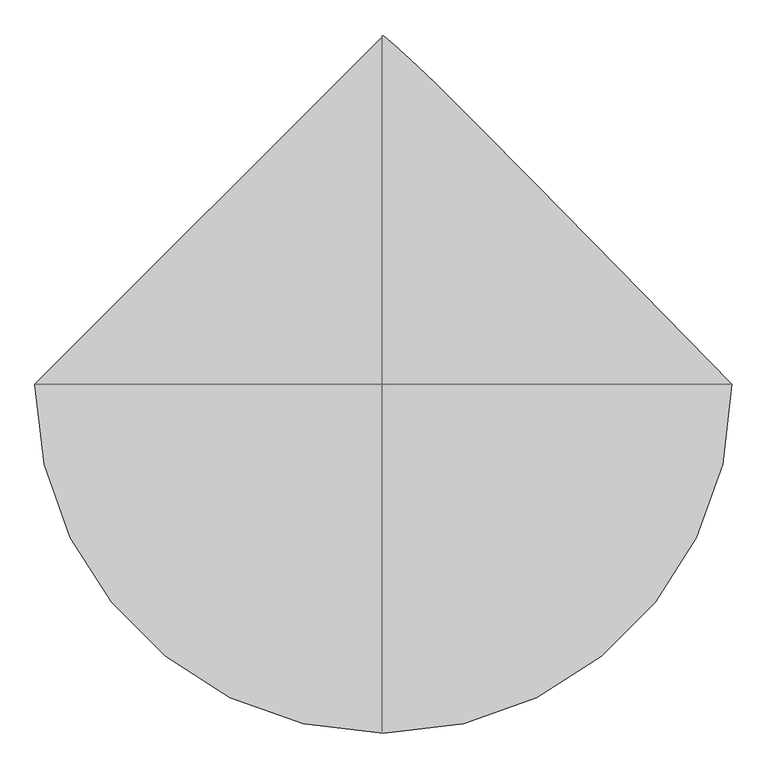
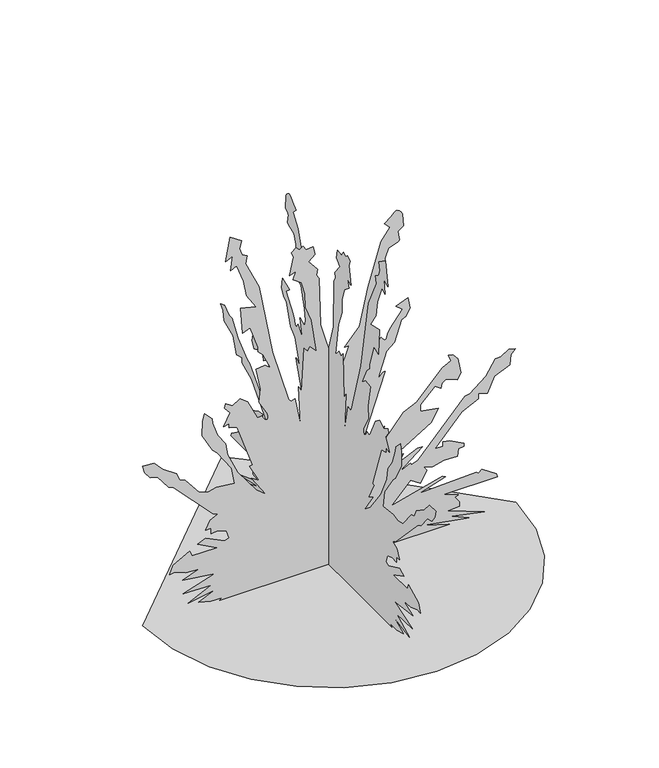
"""IFC4 building model written with IfcOpenShell, lengths in millimetres: proxy geometry, maiden grass 26738 : maiden grass 26738."""

from ifc_helpers import new_model, si_unit, origin, place, context, project, spatial, triangles, source, transform, mapped, element, save


def entourage_51d93d44(model_context):
    return source(origin(), model_context, "Body", "Tessellation", [
        triangles([(-822.1126825, 0.0, 0.0001374), (-800.3786167, -188.373858, 0.0001374), (-738.480578, -361.3651156, 0.0001374), (-641.3745867, -514.0173532, 0.0001374), (-514.0174622, -641.374732, 0.0001374), (-361.365043, -738.4805054, 0.0001374), (-188.3737671, -800.378544, 0.0001374), (3.59e-05, -822.1126825, 0.0001374), (188.3739125, -800.3786167, 0.0001374), (361.3651883, -738.480578, 0.0001374), (514.0174622, -641.3745867, 0.0001374), (641.3748047, -514.0174622, 0.0001374), (738.4805054, -361.365043, 0.0001374), (800.378544, -188.373749, 0.0001374), (822.1126825, 7.19e-05, 0.0001374), (554.9441065, 274.0493697, 0.0001374), (356.8788342, 475.8195757, 0.0001374), (216.3996546, 617.3571573, 0.0001374), (121.9894107, 710.7087994, 0.0001374), (62.1308551, 767.9210049, 0.0001374), (25.3067606, 801.0401316, 0.0001374), (-0.0001078, 822.1126825, 0.0001374), (-486.0236403, 7.81e-05, 0.9155915), (-471.7920599, 7.76e-05, 9.8343198), (-523.9165309, 7.76e-05, 9.7573804), (-575.3383922, 7.67e-05, 24.6529329), (-504.1805263, 7.48e-05, 56.6647099), (-622.6670803, 7.61e-05, 35.566252), (-521.099806, 7.32e-05, 83.8197293), (-644.3685173, 7.29e-05, 88.7502968), (-506.307395, 7.03e-05, 133.1254316), (-645.8895727, 6.92e-05, 151.363835), (-575.3383922, 6.76e-05, 177.5005391), (-633.4720894, 6.73e-05, 182.811861), (-682.2468012, 6.62e-05, 200.8128698), (-703.5376528, 6.64e-05, 197.2227365), (-688.7453144, 6.41e-05, 236.667331), (-614.7840586, 6.17e-05, 276.1118528), (-604.9224512, 6.32e-05, 251.4590335), (-494.8790591, 6.34e-05, 248.9685605), (-580.2687962, 6.06e-05, 295.8341047), (-545.7534247, 5.97e-05, 310.6258072), (-461.9305979, 6.2e-05, 271.1812672), (-442.4802589, 6.16e-05, 277.8612192), (-452.1878423, 5.96e-05, 312.2414789), (-492.5862848, 5.87e-05, 327.4185685), (-520.7920123, 5.89e-05, 323.5701842), (-521.099806, 5.73e-05, 350.0703109), (-545.7534247, 5.73e-05, 350.0703109), (-526.0308277, 5.5e-05, 389.5148872), (-491.515202, 5.41e-05, 404.3065716), (-513.2632931, 5.35e-05, 414.7085166), (-685.7770363, 4.26e-05, 596.5231456), (-707.8857159, 4.2e-05, 606.6573017), (-757.7759846, 3.82e-05, 670.5571804), (-790.6316099, 3.78e-05, 677.9690826), (-814.6804327, 3.58e-05, 711.7275599), (-821.8761417, 3.38e-05, 744.5156021), (-771.5802292, 3.4e-05, 740.8769434), (-734.9066683, 3.66e-05, 698.0076851), (-673.9536301, 3.91e-05, 655.7654961), (-659.1609283, 4.12e-05, 621.2515417), (-636.2393623, 4.16e-05, 613.9256081), (-573.062332, 4.63e-05, 535.429927), (-531.2541281, 4.7e-05, 522.9600486), (-496.445933, 4.65e-05, 532.501254), (-417.5538008, 4.7e-05, 522.6401553), (-431.8794525, 4.26e-05, 597.7539207), (-494.1621334, 3.7e-05, 691.4321417), (-515.1618327, 3.58e-05, 710.6897598), (-560.6032451, 3.08e-05, 794.7286709), (-559.6332461, 2.68e-05, 861.8978268), (-550.6847371, 2.5e-05, 892.4327362), (-516.1688933, 2.71e-05, 857.9187092), (-514.4276842, 2.84e-05, 836.1371899), (-492.5786181, 3.21e-05, 773.1969183), (-456.9999032, 3.53e-05, 719.8628918), (-448.1073864, 3.85e-05, 666.0661755), (-403.8973306, 4.42e-05, 569.7717261), (-322.5198123, 5.08e-05, 459.5990905), (-279.4932235, 5.29e-05, 424.0288053), (-341.7963246, 4.73e-05, 518.5882951), (-309.0772825, 4.85e-05, 497.987336), (-351.6489936, 4.37e-05, 579.3482491), (-338.6617049, 4.35e-05, 581.8069654), (-407.6923751, 3.18e-05, 779.0296291), (-442.2077102, 3.12e-05, 788.8907278), (-442.2077102, 3e-05, 808.6129978), (-466.8613289, 3.03e-05, 803.6824848), (-437.2769065, 2.71e-05, 857.9187092), (-461.9305979, 2.53e-05, 887.5020779), (-456.9999032, 2.41e-05, 907.2244205), (-427.4157715, 2.53e-05, 887.5020779), (-392.9001457, 2.41e-05, 907.2244205), (-361.3909862, 2.55e-05, 883.444622), (-319.5289701, 3.13e-05, 794.863619), (-316.5251201, 3.15e-05, 792.847681), (-312.9193082, 3.15e-05, 792.290593), (-308.9018935, 3.15e-05, 792.6843916), (-304.6633259, 3.13e-05, 793.5212591), (-300.3935829, 3.11e-05, 794.293523), (-296.2831507, 3.08e-05, 794.4932928), (-293.8821344, 3.1e-05, 789.7024515), (-291.6524922, 3.11e-05, 784.6016001), (-289.2939152, 3.13e-05, 779.6455799), (-286.5060222, 3.14e-05, 775.2894505), (-282.9887042, 3.16e-05, 771.9882711), (-278.4414163, 3.19e-05, 770.1969561), (-272.5639226, 3.23e-05, 770.3705647), (-270.4821274, 3.19e-05, 776.4802935), (-269.746798, 3.16e-05, 782.5422054), (-271.4178988, 3.09e-05, 794.5538269), (-309.0772825, 2.68e-05, 862.8492222), (-304.1468967, 2.32e-05, 922.0159595), (-323.8695119, 1.74e-05, 1020.6273823), (-284.423464, 1.71e-05, 1025.5578953), (-259.7697544, 1.82e-05, 1005.8357706), (-292.5143764, 1.4e-05, 1076.7667608), (-314.0080499, 1.27e-05, 1099.5164623), (-315.0547156, 1.15e-05, 1119.0795851), (-348.5233486, 5.3e-06, 1222.7807407), (-383.038502, 6.2e-06, 1207.9888384), (-391.1781941, -1e-06, 1327.8346481), (-323.8695119, 0.0, 1311.5309921), (-365.2547038, -3.9e-06, 1377.9884182), (-377.5616561, -8.2e-06, 1449.0455635), (-409.7759325, -1.31e-05, 1532.0531422), (-435.1933854, -1.24e-05, 1519.3450516), (-427.4157715, -1.61e-05, 1582.7118233), (-456.9999032, -1.53e-05, 1567.9204296), (-438.6445556, -2.17e-05, 1676.3998547), (-387.9694147, -1.97e-05, 1641.8788513), (-396.0815286, -1.75e-05, 1605.9381672), (-384.2218237, -1.56e-05, 1574.3406773), (-363.3155416, -1.5e-05, 1562.9896259), (-368.246309, -1.29e-05, 1528.4758896), (-309.0772825, -5.3e-06, 1400.2812435), (-250.6196225, 1.42e-05, 1073.5192846), (-180.2010283, 2.87e-05, 830.6251717), (-169.6161911, 2.95e-05, 817.4087545), (-151.2930636, 2.91e-05, 823.4046822), (-126.6192335, 3.68e-05, 694.4196774), (-136.5008433, 2.62e-05, 872.7103935), (-121.7086412, 2.76e-05, 848.0576105), (-111.8470156, 1.59e-05, 1045.2803106), (-97.0548044, 1.71e-05, 1025.5578953), (-84.6295182, 1.62e-05, 1040.6290684), (-57.6092516, 1.79e-05, 1010.7662109), (-79.5582798, 8.8e-06, 1163.7574539), (-104.4511553, 4.7e-06, 1232.6419121), (-107.5404289, 9e-07, 1296.0368797), (-123.4986664, -2.4e-06, 1352.177639), (-161.1545347, -4.1e-06, 1380.5586102), (-146.3623326, -6.2e-06, 1415.0727825), (-175.9469094, -5.6e-06, 1405.2116112), (-158.7234512, -1.03e-05, 1484.8167812), (-166.0854474, -1.17e-05, 1508.7534016), (-146.3623326, -1.26e-05, 1523.5452312), (-131.5704484, -1.17e-05, 1508.7534016), (-116.6065998, -1.25e-05, 1521.4754448), (-101.9855355, -1.11e-05, 1498.8923756), (-72.4009586, -1.14e-05, 1503.8230339), (-62.5394784, -9.1e-06, 1464.3783485), (-92.1240644, -7.6e-06, 1439.7256382), (-52.6780073, -4.7e-06, 1390.4200722), (-57.6092516, -3.2e-06, 1365.7670712), (-44.9584885, -2.1e-06, 1346.546006), (-40.1288097, 1.1e-05, 1128.143712), (16.3521246, 2.24e-05, 936.8077166), (25.6302442, 2.16e-05, 950.3199005), (46.3616142, 2.59e-05, 877.5758669), (85.383115, 1.94e-05, 986.1135006), (65.6596505, 1.94e-05, 986.1135006), (132.852038, 1.49e-05, 1062.0039265), (169.7376772, 4.9e-06, 1229.8971668), (228.245861, -6.6e-06, 1421.9566647), (267.8211162, -9.7e-06, 1474.2395199), (243.1672431, -1.11e-05, 1498.8923756), (272.0833378, -1.25e-05, 1521.3225471), (286.4673436, -1.31e-05, 1537.556876), (293.7374485, -1.35e-05, 1542.3155972), (297.4055931, -1.38e-05, 1543.2675739), (308.1376596, -1.27e-05, 1537.579549), (315.8437663, -1.16e-05, 1529.0826839), (321.0283699, -1.07e-05, 1518.2452641), (326.6370392, -7.7e-06, 1460.8509476), (306.7311321, -7.7e-06, 1447.4507481), (304.3311514, -7.7e-06, 1444.519241), (302.7936726, -7.7e-06, 1441.4505329), (309.1859605, -6.2e-06, 1402.4600349), (307.1584316, -5.9e-06, 1398.4450184), (302.9130694, -5.6e-06, 1394.7411747), (261.356885, -4e-06, 1379.0709103), (246.0123274, -1.6e-06, 1337.9506004), (244.0019305, 9e-07, 1296.3149151), (228.3094291, 3.3e-06, 1256.0202816), (220.8882069, 7.9e-06, 1179.9705631), (207.4437332, 6.8e-06, 1171.8723656), (179.3911032, 1.38e-05, 1079.9680189), (173.3980279, 1.7e-05, 1026.8490955), (180.4457445, 1.86e-05, 999.5491631), (213.582312, 1.77e-05, 1015.6967239), (193.859715, 2.26e-05, 931.8771309), (228.3750501, 2e-05, 976.2522566), (242.287573, 2.11e-05, 957.5074705), (251.845438, 2.09e-05, 961.1874784), (256.8526723, 1.97e-05, 980.8979033), (266.7142615, 1.85e-05, 1002.0413801), (322.059448, 1.41e-05, 1074.863534), (293.6769507, 1.28e-05, 1097.3908653), (346.713212, 1.15e-05, 1119.2386597), (354.6484835, 1.44e-05, 1069.6418324), (338.174271, 1.65e-05, 1035.8738354), (317.1287169, 1.71e-05, 1025.5578953), (287.5436224, 2.26e-05, 931.8771309), (252.1265254, 2.44e-05, 903.2333851), (213.582312, 3.12e-05, 788.8907278), (236.8349806, 3.03e-05, 809.7009401), (240.9621815, 3e-05, 811.6948591), (244.803971, 2.97e-05, 812.5061468), (244.8585279, 3e-05, 809.5433916), (134.690634, 4.91e-05, 488.1261283), (242.8606121, 4.5e-05, 557.2269977), (237.4122891, 4.6e-05, 540.8212403), (140.9250282, 5.13e-05, 450.6353934), (129.759903, 5.23e-05, 433.8900129), (164.2748021, 5.06e-05, 463.4733816), (174.1367001, 5.06e-05, 463.4733816), (159.0154937, 5.29e-05, 425.0493098), (238.8042827, 4.92e-05, 486.724506), (326.990179, 4.29e-05, 591.668064), (382.9130736, 4.13e-05, 618.7366516), (499.039125, 3.41e-05, 739.7414022), (534.9049227, 3.29e-05, 759.6449112), (524.2203278, 3.12e-05, 788.8907278), (544.510332, 3.15e-05, 783.3986212), (566.5761726, 3.31e-05, 756.7437075), (580.5672881, 3.72e-05, 688.0601091), (563.6663939, 3.88e-05, 660.6960091), (514.5438108, 3.76e-05, 681.3525244), (496.7209162, 3.83e-05, 668.9436161), (492.0994686, 3.96e-05, 646.9967726), (465.0513376, 3.85e-05, 665.6265947), (400.9515075, 4.23e-05, 601.5291627), (400.9515075, 4.41e-05, 571.9458303), (479.8436033, 4.5e-05, 557.154146), (450.2590719, 4.82e-05, 502.9179216), (287.5436224, 5.41e-05, 404.3065716), (325.8399585, 5.44e-05, 399.649116), (302.3363241, 5.64e-05, 364.8620679), (387.4521134, 5.41e-05, 404.7523293), (411.1211992, 5.41e-05, 403.6902938), (307.2671459, 5.91e-05, 320.4869785), (356.5747104, 5.76e-05, 345.1397979), (361.5048964, 5.82e-05, 335.2785539), (389.4130039, 5.74e-05, 348.2994524), (598.1816563, 4.41e-05, 571.9458303), (618.663909, 4.38e-05, 576.9850576), (688.6817282, 4.05e-05, 633.1896212), (731.3115389, 3.65e-05, 700.1405491), (755.9652666, 3.65e-05, 700.1405491), (790.4811104, 3.5e-05, 724.7934048), (820.0657145, 3.56e-05, 714.9323061), (800.3426451, 3.68e-05, 695.2100361), (795.4119141, 3.94e-05, 650.8349104), (726.3813166, 4.12e-05, 621.2515417), (696.7968578, 4.53e-05, 552.2235603), (657.3502831, 4.47e-05, 562.084659), (657.4310921, 4.61e-05, 538.9833801), (583.1111009, 4.8e-05, 506.1758986), (465.0513376, 5.59e-05, 374.7231666), (499.5666, 5.59e-05, 374.7231666), (499.5666, 5.47e-05, 394.4454366), (528.894134, 5.5e-05, 389.8867032), (593.2509616, 5.7e-05, 355.0009329), (593.2509616, 5.79e-05, 340.2092485), (568.4129791, 5.81e-05, 337.6585321), (563.6663939, 6e-05, 305.6952579), (504.8713271, 5.99e-05, 306.2484581), (453.6921109, 6.06e-05, 295.5878443), (415.7437732, 6e-05, 305.6952579), (430.5360752, 6.11e-05, 285.9729515), (400.9515075, 6.41e-05, 236.667331), (356.5747104, 6.23e-05, 266.2507178), (272.7518472, 6.76e-05, 177.5005391), (498.0560818, 6.42e-05, 234.1173413), (512.2016573, 6.46e-05, 227.2681409), (396.0207401, 6.67e-05, 192.2922235), (647.8657602, 6.62e-05, 201.1622852), (657.3502831, 6.67e-05, 192.2922235), (672.1430574, 6.59e-05, 207.083926), (736.2428513, 6.85e-05, 162.7088003), (741.1735823, 6.94e-05, 147.9171159), (499.5666, 6.94e-05, 147.9171159), (568.5971612, 7.08e-05, 123.2642602), (552.2703235, 7.12e-05, 117.9041314), (573.5278922, 7.29e-05, 88.7502968), (573.5278922, 7.41e-05, 69.0280223), (521.428892, 7.43e-05, 64.9850141), (682.0040108, 7.79e-05, 4.9306691), (539.0127025, 7.61e-05, 34.5140656), (617.9047256, 7.82e-05, 0.0001036), (415.7437732, 7.61e-05, 34.5140656), (529.1511314, 7.82e-05, 0.0001036), (-3.5682026, -482.4553988, 0.9154881), (-3.5682026, -468.2238184, 9.8342176), (-3.5682026, -520.3482894, 9.7572771), (-3.5682026, -571.770187, 24.652833), (-3.5682026, -500.6122484, 56.6646145), (-3.5682026, -619.0989115, 35.5661476), (-3.5682026, -517.5314919, 83.8196294), (-3.5682026, -640.8002758, 88.750206), (-3.5682026, -502.7391898, 133.1253407), (-3.5682026, -642.3213312, 151.3637533), (-3.5682026, -571.770187, 177.5004483), (-3.5682026, -629.9037752, 182.8117702), (-3.5682026, -678.6785597, 200.8127971), (-3.5682026, -699.9694839, 197.2226638), (-3.5682026, -685.1770729, 236.6672583), (-3.5682026, -611.2158897, 276.1117802), (-3.5682026, -601.3542097, 251.4589427), (-3.5682026, -491.310854, 248.9684878), (-3.5682026, -576.7005547, 295.8340138), (-3.5682026, -542.1852559, 310.6257345), (-3.5682026, -458.3623564, 271.1812308), (-3.5682026, -438.9119811, 277.8611647), (-3.5682026, -448.6196008, 312.2414426), (-3.5682026, -489.0179707, 327.4185322), (-3.5682026, -517.2238071, 323.5701479), (-3.5682026, -517.5314919, 350.0702745), (-3.5682026, -542.1852559, 350.0702745), (-3.5682026, -522.4626225, 389.5148509), (-3.5682026, -487.9469604, 404.3065352), (-3.5682026, -509.6950516, 414.7084803), (-3.5682026, -682.2087948, 596.5231456), (-3.5682026, -704.3174744, 606.6573017), (-3.5682026, -754.2077431, 670.5571804), (-3.5682026, -787.0633684, 677.9690826), (-3.5682026, -811.1121912, 711.7275599), (-3.5682026, -818.3079729, 744.5156021), (-3.5682026, -768.0119877, 740.8769434), (-3.5682026, -731.3384995, 698.0076851), (-3.5682026, -670.3853886, 655.7654961), (-3.5682026, -655.5926868, 621.251469), (-3.5682026, -632.6711208, 613.9256081), (-3.5682026, -569.4940905, 535.4298543), (-3.5682026, -527.6859229, 522.9599759), (-3.5682026, -492.8777278, 532.501254), (-3.5682026, -413.9855593, 522.6401553), (-3.5682026, -428.311211, 597.7538844), (-3.5682026, -490.5938556, 691.4321417), (-3.5682026, -511.5936275, 710.6897598), (-3.5682026, -557.0350036, 794.7286709), (-3.5682026, -556.0649683, 861.8978268), (-3.5682026, -547.1164956, 892.4327362), (-3.5682026, -512.6006518, 857.9187092), (-3.5682026, -510.85937, 836.1371899), (-3.5682026, -489.0103766, 773.1969183), (-3.5682026, -453.4316254, 719.8628918), (-3.5682026, -444.5391449, 666.0661028), (-3.5682026, -400.3290891, 569.7716535), (-3.5682026, -318.9515708, 459.5990541), (-3.5682026, -275.9250001, 424.0287689), (-3.5682026, -338.2281195, 518.5882224), (-3.5682026, -305.5090774, 497.9872996), (-3.5682026, -348.0807884, 579.3482491), (-3.5682026, -335.0934634, 581.8069654), (-3.5682026, -404.1241336, 779.0296291), (-3.5682026, -438.6394687, 788.8907278), (-3.5682026, -438.6394687, 808.6129978), (-3.5682026, -463.2930874, 803.6824848), (-3.5682026, -433.7087377, 857.9187092), (-3.5682026, -458.3623564, 887.5020779), (-3.5682026, -453.4316254, 907.2244205), (-3.5682026, -423.84753, 887.5020779), (-3.5682026, -389.3319042, 907.2244205), (-3.5682026, -357.8227083, 883.444622), (-3.5682026, -315.9607286, 794.863619), (-3.5682026, -312.9568422, 792.847681), (-3.5682026, -309.351103, 792.290593), (-3.5682026, -305.3336884, 792.6843916), (-3.5682026, -301.0950844, 793.5212591), (-3.5682026, -296.8253414, 794.293523), (-3.5682026, -292.7149092, 794.4932928), (-3.5682026, -290.3138929, 789.7024515), (-3.568202, -288.0842507, 784.6016001), (-3.568202, -285.7257101, 779.6455799), (-3.568202, -282.9377988, 775.2894505), (-3.568202, -279.4204808, 771.9882711), (-3.568202, -274.873193, 770.1969561), (-3.5682026, -268.9956993, 770.3705647), (-3.5682026, -266.9138678, 776.4802935), (-3.5682026, -266.1785747, 782.5422054), (-3.5682026, -267.8496573, 794.5538269), (-3.5682026, -305.5090774, 862.8492222), (-3.5682026, -300.5786552, 922.0161776), (-3.5682026, -320.3012704, 1020.6273823), (-3.5682026, -280.8552043, 1025.5579679), (-3.5682026, -256.2015129, 1005.8357706), (-3.5682026, -288.946153, 1076.7667608), (-3.5682026, -310.4398084, 1099.5164623), (-3.5682026, -311.4864741, 1119.0795851), (-3.5682026, -344.9551071, 1222.7807407), (-3.5682026, -379.4702605, 1207.9888384), (-3.5682026, -387.6099526, 1327.8347935), (-3.5682026, -320.3012704, 1311.5309921), (-3.5682026, -361.6864986, 1377.9885635), (-3.5682026, -373.9934146, 1449.0455635), (-3.5682026, -406.2076547, 1532.0531422), (-3.5682026, -431.6251802, 1519.3451969), (-3.5682026, -423.84753, 1582.712114), (-3.5682026, -453.4316254, 1567.9204296), (-3.5682026, -435.0763867, 1676.4), (-3.5682026, -384.4011732, 1641.8788513), (-3.5682026, -392.5132507, 1605.9383125), (-3.5682026, -380.6535822, 1574.3408226), (-3.5682026, -359.7473365, 1562.9896259), (-3.5682026, -364.6781038, 1528.4760349), (-3.5682026, -305.5090774, 1400.2812435), (-3.5682026, -247.0513992, 1073.5192846), (-3.5682026, -176.632805, 830.6251717), (-3.5682026, -166.0479678, 817.4087545), (-3.5682026, -147.7248221, 823.4047548), (-3.5682026, -123.0510011, 694.4196774), (-3.5682026, -132.93262, 872.7103935), (-3.5682026, -118.1404088, 848.0576105), (-3.5682026, -108.2787832, 1045.2803833), (-3.5682026, -93.486572, 1025.5579679), (-3.5682026, -81.0612858, 1040.6290684), (-3.5682026, -54.0410146, 1010.7662109), (-3.5682026, -75.9900428, 1163.7574539), (-3.5682026, -100.8829229, 1232.6419121), (-3.5682026, -103.9721874, 1296.0368797), (-3.5682026, -119.9304249, 1352.177639), (-3.5682026, -157.5863113, 1380.5587555), (-3.5682026, -142.7940911, 1415.0729279), (-3.5682026, -172.3786679, 1405.2117565), (-3.5682026, -155.1552097, 1484.8169266), (-3.5682026, -162.517224, 1508.7536922), (-3.5682026, -142.7940911, 1523.5453766), (-3.5682026, -128.002225, 1508.7536922), (-3.5682026, -113.0383673, 1521.4754448), (-3.5682026, -98.417303, 1498.8925209), (-3.5682026, -68.8327217, 1503.8230339), (-3.5682026, -58.9712415, 1464.3784939), (-3.5682026, -88.5558228, 1439.7256382), (-3.5682026, -49.1097749, 1390.4200722), (-3.5682026, -54.0410146, 1365.7670712), (-3.5682026, -41.3902516, 1346.5461514), (-3.5682026, -36.560575, 1128.143712), (-3.5682026, 19.9203638, 936.8078619), (-3.5682026, 29.1984812, 950.3199005), (-3.5682026, 49.9298511, 877.5758669), (-3.5682026, 88.9513474, 986.1135006), (-3.5682026, 69.2278874, 986.1135006), (-3.5682026, 136.4202886, 1062.0039991), (-3.5682026, 173.3059187, 1229.8973122), (-3.5682026, 231.8141025, 1421.95681), (-3.5682026, 271.3893577, 1474.2395199), (-3.5682026, 246.7355028, 1498.8925209), (-3.5682026, 275.6515793, 1521.3226925), (-3.5682026, 290.0355851, 1537.5570213), (-3.5682026, 297.30569, 1542.3158878), (-3.5682026, 300.9738527, 1543.2675739), (-3.5682032, 311.7059011, 1537.5796944), (-3.5682035, 319.4120078, 1529.0828293), (-3.568204, 324.5966477, 1518.2452641), (-3.5682035, 330.2052807, 1460.8509476), (-3.5682026, 310.2993736, 1447.4507481), (-3.5682026, 307.8994111, 1444.5193863), (-3.5682026, 306.3618959, 1441.4505329), (-3.5682015, 312.754202, 1402.4600349), (-3.5682015, 310.7266368, 1398.4451637), (-3.5682015, 306.4812927, 1394.74132), (-3.5682026, 264.9251265, 1379.0710556), (-3.5682026, 249.5805508, 1337.9507458), (-3.5682026, 247.5701539, 1296.3149151), (-3.5682026, 231.8776706, 1256.0204269), (-3.5682026, 224.4564302, 1179.9705631), (-3.5682012, 211.0119747, 1171.8725836), (-3.5682026, 182.9593447, 1079.9680189), (-3.5682026, 176.9662694, 1026.8490955), (-3.5682026, 184.0139678, 999.5491631), (-3.5682026, 217.1505535, 1015.6968693), (-3.5682026, 197.4279383, 931.8772036), (-3.5682026, 231.9432552, 976.2522566), (-3.5682026, 245.8557963, 957.5075432), (-3.5682026, 255.4136795, 961.1876965), (-3.5682026, 260.4209138, 980.8979033), (-3.5682026, 270.2824848, 1002.0413801), (-3.5682026, 325.6276895, 1074.863534), (-3.5682026, 297.2451922, 1097.3908653), (-3.5682026, 350.2814172, 1119.2386597), (-3.5682026, 358.216725, 1069.6418324), (-3.5682026, 341.7425125, 1035.8738354), (-3.5682026, 320.6969584, 1025.5579679), (-3.5682026, 291.1118639, 931.8772036), (-3.5682026, 255.694767, 903.2333851), (-3.5682026, 217.1505535, 788.8907278), (-3.5682026, 240.4032221, 809.7009401), (-3.5682026, 244.5303866, 811.6948591), (-3.5682026, 248.3722125, 812.5061468), (-3.5682026, 248.4268058, 809.5433916), (-3.5682026, 138.2588664, 488.1261283), (-3.5682026, 246.4288173, 557.2269613), (-3.5682026, 240.9805125, 540.8212403), (-3.5682026, 144.4932697, 450.6353208), (-3.5682026, 133.3281354, 433.8899766), (-3.5682026, 167.8430436, 463.4733089), (-3.5682026, 177.7049234, 463.4733089), (-3.5682026, 162.5837171, 425.0492735), (-3.5682026, 242.3725242, 486.724397), (-3.5682026, 330.5584205, 591.668064), (-3.5682026, 386.4813151, 618.7366516), (-3.5682026, 502.6072938, 739.7414022), (-3.5682026, 538.4731278, 759.6449112), (-3.5682026, 527.7886419, 788.8907278), (-3.5682026, 548.0786098, 783.3986212), (-3.5682026, 570.1443778, 756.7437075), (-3.5682026, 584.1354933, 688.0601091), (-3.5682026, 567.2346717, 660.6960091), (-3.5682026, 518.112016, 681.3525244), (-3.5682026, 500.2891577, 668.9436161), (-3.5682026, 495.6677828, 646.9966999), (-3.5682026, 468.6195791, 665.6265947), (-3.5682026, 404.519749, 601.5291264), (-3.5682026, 404.519749, 571.9457577), (-3.5682026, 483.4118448, 557.1540733), (-3.5682026, 453.8273134, 502.917849), (-3.5682026, 291.1118639, 404.3065352), (-3.5682026, 329.4082363, 399.6490434), (-3.5682026, 305.9045837, 364.8620316), (-3.5682026, 391.0203549, 404.7522566), (-3.5682026, 414.6894407, 403.6902211), (-3.5682026, 310.8353874, 320.4869059), (-3.5682026, 360.1429519, 345.1397615), (-3.5682026, 365.0731379, 335.2785539), (-3.5682026, 392.9812454, 348.2994161), (-3.5682026, 601.7499341, 571.9457577), (-3.5682026, 622.2321505, 576.9850576), (-3.5682026, 692.2499697, 633.1895485), (-3.5682026, 734.8797804, 700.1405491), (-3.5682026, 759.5335808, 700.1405491), (-3.5682026, 794.0494246, 724.7934048), (-3.5682026, 823.6338106, 714.9323061), (-3.5682026, 803.9108866, 695.2100361), (-3.5682026, 798.9800829, 650.8349104), (-3.5682026, 729.9495581, 621.251469), (-3.5682026, 700.3650267, 552.223524), (-3.5682026, 660.9185246, 562.084659), (-3.5682026, 660.9993336, 538.9833801), (-3.5682026, 586.679306, 506.175826), (-3.5682026, 468.6195791, 374.7231302), (-3.5682026, 503.1348415, 374.7231302), (-3.5682026, 503.1348415, 394.4453639), (-3.5682026, 532.4624119, 389.8866669), (-3.5682026, 596.8191668, 355.0008602), (-3.5682026, 596.8191668, 340.2091759), (-3.5682026, 571.981257, 337.6584958), (-3.5682026, 567.2346717, 305.6951852), (-3.5682026, 508.4395686, 306.2483854), (-3.5682026, 457.2603161, 295.5877898), (-3.5682026, 419.3120147, 305.6951852), (-3.5682026, 434.1043167, 285.9729152), (-3.5682026, 404.519749, 236.6672583), (-3.5682026, 360.1429519, 266.2506452), (-3.5682026, 276.3200705, 177.5004483), (-3.5682026, 501.6243959, 234.1172686), (-3.5682026, 515.7698625, 227.2680864), (-3.5682026, 399.5889816, 192.2921508), (-3.5682026, 651.4340017, 201.1622126), (-3.5682026, 660.9185246, 192.2921508), (-3.5682026, 675.7112989, 207.0838533), (-3.5682026, 739.8110928, 162.7087094), (-3.5682026, 744.7418238, 147.9170433), (-3.5682026, 503.1348415, 147.9170433), (-3.5682026, 572.1653664, 123.2641785), (-3.5682026, 555.8386013, 117.9040406), (-3.5682026, 577.0961337, 88.750206), (-3.5682026, 577.0961337, 69.027936), (-3.5682026, 524.9970972, 64.9849233), (-3.5682026, 685.5723249, 4.9305664), (-3.5682026, 542.5808713, 34.5139657), (-3.5682026, 621.4728945, 0.0), (-3.5682026, 419.3120147, 34.5139657), (-3.5682026, 532.7193003, 0.0)], [[21, 22, 1], [20, 21, 1], [19, 20, 1], [18, 19, 1], [17, 18, 1], [17, 1, 2], [17, 2, 3], [17, 3, 4], [16, 17, 4], [16, 4, 5], [16, 5, 6], [16, 6, 7], [16, 7, 8], [16, 8, 9], [16, 9, 10], [16, 10, 11], [16, 11, 12], [15, 16, 12], [14, 15, 12], [13, 14, 12], [299, 300, 301], [301, 302, 303], [27, 28, 29], [303, 304, 23], [29, 30, 31], [81, 82, 83], [31, 32, 33], [142, 143, 144], [303, 23, 24], [294, 295, 296], [222, 223, 224], [144, 145, 146], [25, 26, 27], [251, 252, 253], [250, 251, 253], [286, 287, 288], [285, 286, 288], [222, 224, 225], [172, 173, 174], [88, 89, 90], [169, 170, 171], [201, 202, 203], [40, 41, 42], [40, 42, 43], [129, 130, 131], [129, 131, 132], [129, 132, 133], [234, 235, 236], [154, 155, 156], [127, 128, 129], [35, 36, 37], [299, 301, 303], [209, 210, 211], [209, 211, 212], [72, 73, 74], [234, 236, 237], [248, 249, 250], [262, 263, 264], [48, 49, 50], [24, 25, 27], [241, 242, 243], [292, 293, 294], [227, 228, 229], [226, 227, 229], [91, 92, 93], [90, 91, 93], [121, 122, 123], [121, 123, 124], [245, 246, 247], [261, 262, 264], [209, 212, 213], [208, 209, 213], [208, 213, 214], [208, 214, 215], [207, 208, 215], [206, 207, 215], [83, 84, 85], [57, 58, 59], [129, 133, 134], [127, 129, 134], [203, 204, 205], [206, 215, 216], [205, 206, 216], [203, 205, 216], [219, 220, 221], [272, 273, 274], [146, 147, 148], [144, 146, 148], [159, 160, 161], [140, 141, 142], [177, 178, 179], [46, 47, 48], [37, 38, 39], [71, 72, 74], [71, 74, 75], [71, 75, 76], [70, 71, 76], [70, 76, 77], [69, 70, 77], [69, 77, 78], [68, 69, 78], [68, 78, 79], [67, 68, 79], [67, 79, 80], [245, 247, 248], [114, 115, 116], [114, 116, 117], [282, 283, 284], [281, 282, 284], [56, 57, 59], [56, 59, 60], [55, 56, 60], [35, 37, 39], [34, 35, 39], [33, 34, 39], [33, 39, 40], [31, 33, 40], [253, 254, 255], [261, 264, 265], [261, 265, 266], [260, 261, 266], [259, 260, 266], [259, 266, 267], [258, 259, 267], [258, 267, 268], [127, 134, 135], [127, 135, 136], [126, 127, 136], [126, 136, 137], [125, 126, 137], [124, 125, 137], [124, 137, 138], [121, 124, 138], [120, 121, 138], [119, 120, 138], [118, 119, 138], [117, 118, 138], [117, 138, 139], [114, 117, 139], [113, 114, 139], [112, 113, 139], [297, 298, 299], [296, 297, 299], [294, 296, 299], [294, 299, 303], [161, 162, 163], [161, 163, 164], [55, 60, 61], [54, 55, 61], [54, 61, 62], [53, 54, 62], [52, 53, 62], [52, 62, 63], [52, 63, 64], [52, 64, 65], [275, 276, 277], [274, 275, 277], [52, 65, 66], [52, 66, 67], [51, 52, 67], [51, 67, 80], [203, 216, 217], [277, 278, 279], [274, 277, 279], [272, 274, 279], [271, 272, 279], [271, 279, 280], [271, 280, 281], [157, 158, 159], [156, 157, 159], [238, 239, 240], [237, 238, 240], [234, 237, 240], [233, 234, 240], [290, 291, 292], [290, 292, 294], [289, 290, 294], [288, 289, 294], [288, 294, 303], [288, 303, 24], [285, 288, 24], [112, 139, 140], [112, 140, 142], [111, 112, 142], [110, 111, 142], [109, 110, 142], [152, 153, 154], [218, 219, 221], [217, 218, 221], [217, 221, 222], [86, 87, 88], [48, 50, 51], [46, 48, 51], [46, 51, 80], [45, 46, 80], [45, 80, 81], [44, 45, 81], [233, 240, 241], [233, 241, 243], [233, 243, 244], [232, 233, 244], [231, 232, 244], [231, 244, 245], [231, 245, 248], [230, 231, 248], [229, 230, 248], [258, 268, 269], [258, 269, 270], [257, 258, 270], [256, 257, 270], [256, 270, 271], [256, 271, 281], [256, 281, 284], [255, 256, 284], [253, 255, 284], [253, 284, 285], [285, 24, 27], [253, 285, 27], [250, 253, 27], [248, 250, 27], [229, 248, 27], [226, 229, 27], [226, 27, 29], [226, 29, 31], [226, 31, 40], [226, 40, 43], [226, 43, 44], [226, 44, 81], [226, 81, 83], [93, 94, 95], [90, 93, 95], [88, 90, 95], [86, 88, 95], [85, 86, 95], [85, 95, 96], [85, 96, 97], [85, 97, 98], [85, 98, 99], [85, 99, 100], [85, 100, 101], [85, 101, 102], [85, 102, 103], [85, 103, 104], [85, 104, 105], [85, 105, 106], [85, 106, 107], [85, 107, 108], [85, 108, 109], [85, 109, 142], [83, 85, 142], [226, 83, 142], [225, 226, 142], [222, 225, 142], [217, 222, 142], [217, 142, 144], [159, 161, 164], [156, 159, 164], [154, 156, 164], [152, 154, 164], [152, 164, 165], [152, 165, 166], [151, 152, 166], [151, 166, 167], [150, 151, 167], [150, 167, 168], [149, 150, 168], [148, 149, 168], [148, 168, 169], [144, 148, 169], [144, 169, 171], [217, 144, 171], [203, 217, 171], [203, 171, 172], [201, 203, 172], [201, 172, 174], [200, 201, 174], [199, 200, 174], [199, 174, 175], [198, 199, 175], [197, 198, 175], [196, 197, 175], [196, 175, 176], [195, 196, 176], [194, 195, 176], [193, 194, 176], [193, 176, 177], [192, 193, 177], [191, 192, 177], [190, 191, 177], [189, 190, 177], [188, 189, 177], [187, 188, 177], [187, 177, 179], [186, 187, 179], [185, 186, 179], [184, 185, 179], [183, 184, 179], [182, 183, 179], [182, 179, 180], [182, 180, 181], [581, 582, 583], [583, 584, 585], [309, 310, 311], [585, 586, 305], [311, 312, 313], [363, 364, 365], [313, 314, 315], [424, 425, 426], [585, 305, 306], [576, 577, 578], [504, 505, 506], [426, 427, 428], [307, 308, 309], [533, 534, 535], [532, 533, 535], [568, 569, 570], [567, 568, 570], [504, 506, 507], [454, 455, 456], [370, 371, 372], [451, 452, 453], [483, 484, 485], [322, 323, 324], [322, 324, 325], [411, 412, 413], [411, 413, 414], [411, 414, 415], [516, 517, 518], [436, 437, 438], [409, 410, 411], [317, 318, 319], [581, 583, 585], [491, 492, 493], [491, 493, 494], [354, 355, 356], [516, 518, 519], [530, 531, 532], [544, 545, 546], [330, 331, 332], [306, 307, 309], [523, 524, 525], [574, 575, 576], [509, 510, 511], [508, 509, 511], [373, 374, 375], [372, 373, 375], [403, 404, 405], [403, 405, 406], [527, 528, 529], [543, 544, 546], [491, 494, 495], [490, 491, 495], [490, 495, 496], [490, 496, 497], [489, 490, 497], [488, 489, 497], [365, 366, 367], [339, 340, 341], [411, 415, 416], [409, 411, 416], [485, 486, 487], [488, 497, 498], [487, 488, 498], [485, 487, 498], [501, 502, 503], [554, 555, 556], [428, 429, 430], [426, 428, 430], [441, 442, 443], [422, 423, 424], [459, 460, 461], [328, 329, 330], [319, 320, 321], [353, 354, 356], [353, 356, 357], [353, 357, 358], [352, 353, 358], [352, 358, 359], [351, 352, 359], [351, 359, 360], [350, 351, 360], [350, 360, 361], [349, 350, 361], [349, 361, 362], [527, 529, 530], [396, 397, 398], [396, 398, 399], [564, 565, 566], [563, 564, 566], [338, 339, 341], [338, 341, 342], [337, 338, 342], [317, 319, 321], [316, 317, 321], [315, 316, 321], [315, 321, 322], [313, 315, 322], [535, 536, 537], [543, 546, 547], [543, 547, 548], [542, 543, 548], [541, 542, 548], [541, 548, 549], [540, 541, 549], [540, 549, 550], [409, 416, 417], [409, 417, 418], [408, 409, 418], [408, 418, 419], [407, 408, 419], [406, 407, 419], [406, 419, 420], [403, 406, 420], [402, 403, 420], [401, 402, 420], [400, 401, 420], [399, 400, 420], [399, 420, 421], [396, 399, 421], [395, 396, 421], [394, 395, 421], [579, 580, 581], [578, 579, 581], [576, 578, 581], [576, 581, 585], [443, 444, 445], [443, 445, 446], [337, 342, 343], [336, 337, 343], [336, 343, 344], [335, 336, 344], [334, 335, 344], [334, 344, 345], [334, 345, 346], [334, 346, 347], [557, 558, 559], [556, 557, 559], [334, 347, 348], [334, 348, 349], [333, 334, 349], [333, 349, 362], [485, 498, 499], [559, 560, 561], [556, 559, 561], [554, 556, 561], [553, 554, 561], [553, 561, 562], [553, 562, 563], [439, 440, 441], [438, 439, 441], [520, 521, 522], [519, 520, 522], [516, 519, 522], [515, 516, 522], [572, 573, 574], [572, 574, 576], [571, 572, 576], [570, 571, 576], [570, 576, 585], [570, 585, 306], [567, 570, 306], [394, 421, 422], [394, 422, 424], [393, 394, 424], [392, 393, 424], [391, 392, 424], [434, 435, 436], [500, 501, 503], [499, 500, 503], [499, 503, 504], [368, 369, 370], [330, 332, 333], [328, 330, 333], [328, 333, 362], [327, 328, 362], [327, 362, 363], [326, 327, 363], [515, 522, 523], [515, 523, 525], [515, 525, 526], [514, 515, 526], [513, 514, 526], [513, 526, 527], [513, 527, 530], [512, 513, 530], [511, 512, 530], [540, 550, 551], [540, 551, 552], [539, 540, 552], [538, 539, 552], [538, 552, 553], [538, 553, 563], [538, 563, 566], [537, 538, 566], [535, 537, 566], [535, 566, 567], [567, 306, 309], [535, 567, 309], [532, 535, 309], [530, 532, 309], [511, 530, 309], [508, 511, 309], [508, 309, 311], [508, 311, 313], [508, 313, 322], [508, 322, 325], [508, 325, 326], [508, 326, 363], [508, 363, 365], [375, 376, 377], [372, 375, 377], [370, 372, 377], [368, 370, 377], [367, 368, 377], [367, 377, 378], [367, 378, 379], [367, 379, 380], [367, 380, 381], [367, 381, 382], [367, 382, 383], [367, 383, 384], [367, 384, 385], [367, 385, 386], [367, 386, 387], [367, 387, 388], [367, 388, 389], [367, 389, 390], [367, 390, 391], [367, 391, 424], [365, 367, 424], [508, 365, 424], [507, 508, 424], [504, 507, 424], [499, 504, 424], [499, 424, 426], [441, 443, 446], [438, 441, 446], [436, 438, 446], [434, 436, 446], [434, 446, 447], [434, 447, 448], [433, 434, 448], [433, 448, 449], [432, 433, 449], [432, 449, 450], [431, 432, 450], [430, 431, 450], [430, 450, 451], [426, 430, 451], [426, 451, 453], [499, 426, 453], [485, 499, 453], [485, 453, 454], [483, 485, 454], [483, 454, 456], [482, 483, 456], [481, 482, 456], [481, 456, 457], [480, 481, 457], [479, 480, 457], [478, 479, 457], [478, 457, 458], [477, 478, 458], [476, 477, 458], [475, 476, 458], [475, 458, 459], [474, 475, 459], [473, 474, 459], [472, 473, 459], [471, 472, 459], [470, 471, 459], [469, 470, 459], [469, 459, 461], [468, 469, 461], [467, 468, 461], [466, 467, 461], [465, 466, 461], [464, 465, 461], [464, 461, 462], [464, 462, 463]], closed=False),
    ])


if __name__ == "__main__":
    model = new_model("IFC4")
    model_context = context("Model", 3, world=origin())
    ifc_project = project(units=[si_unit("LENGTHUNIT", "METRE", prefix="MILLI")], contexts=[model_context])
    site = spatial("IfcSite", under=ifc_project)
    building = spatial("IfcBuilding", under=site)
    placement = place(None, origin())
    entourage_shape = entourage_51d93d44(model_context)
    element("IfcBuildingElementProxy", 1, Name="maiden grass 26738 : maiden grass 26738", ObjectType="maiden grass 26738 : maiden grass 26738", at=placement, inside=building, context=model_context, shape_type="MappedRepresentation", body=[
        mapped(entourage_shape, transform((0.0, 0.0, 0.0), x_axis=(1.0, 0.0, 0.0), y_axis=(0.0, 1.0, 0.0), z_axis=(0.0, 0.0, 1.0))),
    ])
    save(model, "model.ifc")

# Revit data of these elements
# Type "maiden grass 26738 : maiden grass 26738"
#   built-in parameter 1005195 = "RPC-8-G1A1-U7Q0-CHK1-A"
#   Height = 0
